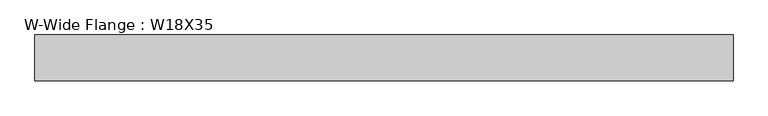
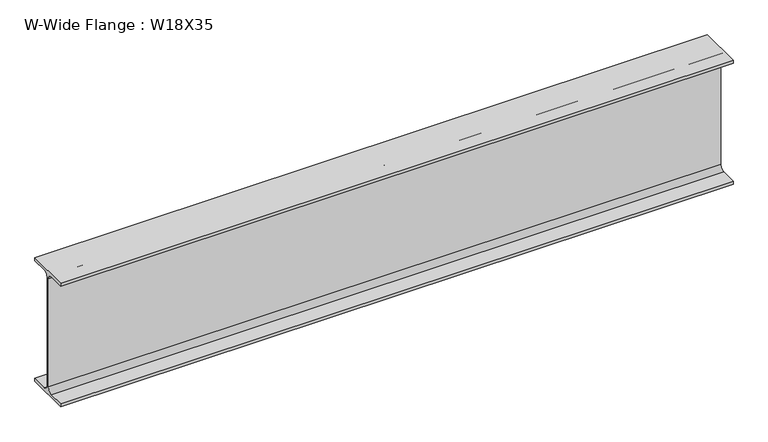
"""IFC4 building model written with IfcOpenShell, lengths in millimetres: beam geometry, W-Wide Flange : W18X35."""

from ifc_helpers import new_model, si_unit, point, frame, frame_2d, origin, place, context, project, spatial, polyline, circle_curve, trimmed, segment, composite_curve, outline, extrude, source, transform, mapped, element, save


def w_wide_flange_w18x35_71e8b52a(model_context):
    return source(origin(), model_context, "Body", "SweptSolid", [
        extrude(outline(composite_curve([segment(polyline([(76.2, -213.995), (76.2, -224.79), (-76.2, -224.79), (-76.2, -213.995), (-21.59, -213.995)]), True, "CONTINUOUS"), segment(trimmed(circle_curve(frame_2d((-21.59, -196.215)), 17.78), [point((-21.59, -213.995))], [point((-3.81, -196.215))], True, "CARTESIAN"), True, "CONTINUOUS"), segment(polyline([(-3.81, -196.215), (-3.81, 196.215)]), True, "CONTINUOUS"), segment(trimmed(circle_curve(frame_2d((-21.59, 196.215)), 17.78), [point((-3.81, 196.215))], [point((-21.59, 213.995))], True, "CARTESIAN"), True, "CONTINUOUS"), segment(polyline([(-21.59, 213.995), (-76.2, 213.995), (-76.2, 224.79), (76.2, 224.79), (76.2, 213.995), (21.59, 213.995)]), True, "CONTINUOUS"), segment(trimmed(circle_curve(frame_2d((21.59, 196.215)), 17.78), [point((21.59, 213.995))], [point((3.81, 196.215))], True, "CARTESIAN"), True, "CONTINUOUS"), segment(polyline([(3.81, 196.215), (3.81, -196.215)]), True, "CONTINUOUS"), segment(trimmed(circle_curve(frame_2d((21.59, -196.215)), 17.78), [point((3.81, -196.215))], [point((21.59, -213.995))], True, "CARTESIAN"), True, "CONTINUOUS"), segment(polyline([(21.59, -213.995), (76.2, -213.995)]), True, "CONTINUOUS")], self_intersect=False)), frame((-1155.7, 0.0, 0.0), z_axis=(1.0, 0.0, 0.0), x_axis=(0.0, 1.0, 0.0)), (0.0, 0.0, 1.0), 2311.4),
    ])


if __name__ == "__main__":
    model = new_model("IFC4")
    model_context = context("Model", 3, world=origin())
    ifc_project = project(units=[si_unit("LENGTHUNIT", "METRE", prefix="MILLI")], contexts=[model_context])
    site = spatial("IfcSite", under=ifc_project)
    building = spatial("IfcBuilding", under=site)
    placement = place(None, origin())
    w_wide_flange_w18x35_shape = w_wide_flange_w18x35_71e8b52a(model_context)
    element("IfcBeam", 1, ObjectType="W-Wide Flange : W18X35", at=placement, inside=building, context=model_context, shape_type="MappedRepresentation", body=[
        mapped(w_wide_flange_w18x35_shape, transform((0.0, 0.0, 0.0), x_axis=(1.0, 0.0, 0.0), y_axis=(0.0, 1.0, 0.0), z_axis=(0.0, 0.0, 1.0))),
    ])
    save(model, "model.ifc")

# Revit data of these elements
# Type "W-Wide Flange : W18X35"
#   Assembly Code = "B10"
#   W = 35
#   Length [instance default] = 5' - 0"
#   bf = 0' - 6"
#   d = 1' - 5.7"
#   k = 0' - 1 1/8"
#   k2 = 0' - 0.7"
#   tf = 0' - 0.425"
#   tw = 0' - 0.3"
#   A = 0.0715278 SF
#   Structural Material [instance default] = Steel ASTM A992
# Element 1 (IfcBeam, "W-Wide Flange : W18X35")
#   Materials on its faces: "Steel ASTM A992"
# Materials
#   "Steel ASTM A992": class "Metal", colour RGB 199 199 199, transparency 0, Description = "Structural steel 50ksi", Cost = 0
